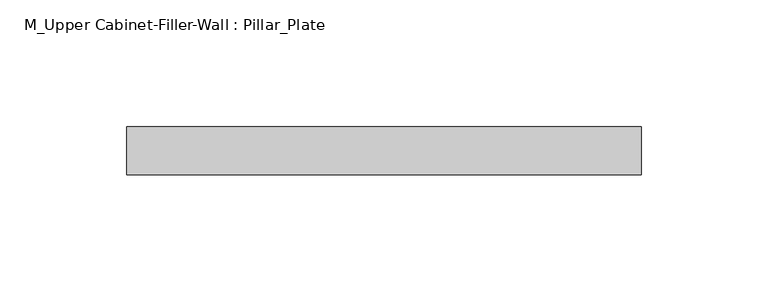
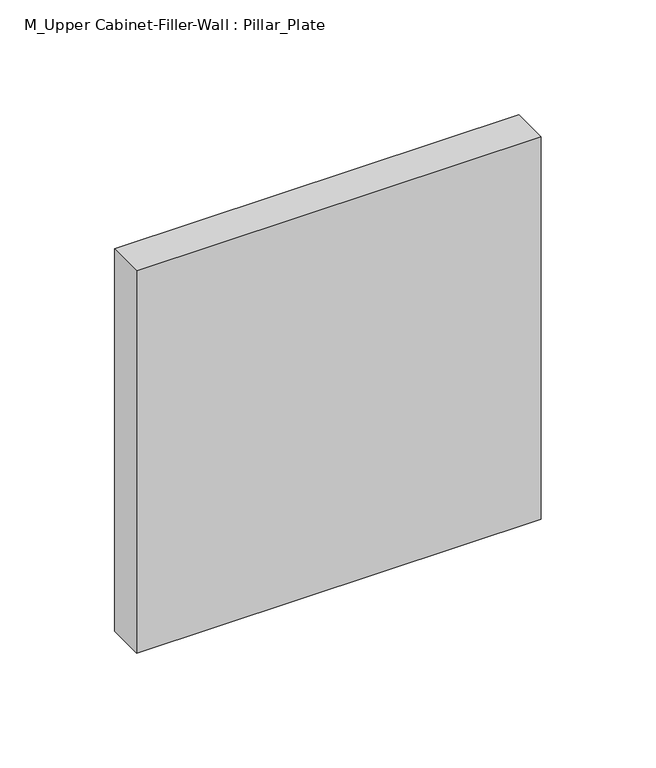
"""IFC4 building model written with IfcOpenShell, lengths in millimetres: furniture geometry, M_Upper Cabinet-Filler-Wall : Pillar_Plate."""

from ifc_helpers import new_model, si_unit, frame, origin, place, context, project, spatial, polyline, outline, extrude, source, transform, mapped, element, save


def m_upper_cabinet_filler_wall_pillar_plate_184ded32(model_context):
    return source(origin(), model_context, "Body", "SweptSolid", [
        extrude(outline(polyline([(-71.8288372, 38.1), (-71.8288372, 57.15), (131.3711628, 57.15), (131.3711628, 38.1), (-71.8288372, 38.1)])), frame((0.0, 0.0, 1796.8), z_axis=(0.0, 0.0, 1.0), x_axis=(1.0, 0.0, 0.0)), (0.0, 0.0, 1.0), 203.2),
    ])


if __name__ == "__main__":
    model = new_model("IFC4")
    model_context = context("Model", 3, world=origin())
    ifc_project = project(units=[si_unit("LENGTHUNIT", "METRE", prefix="MILLI")], contexts=[model_context])
    site = spatial("IfcSite", under=ifc_project)
    building = spatial("IfcBuilding", under=site)
    placement = place(None, origin())
    m_upper_cabinet_filler_wall_pillar_plate_shape = m_upper_cabinet_filler_wall_pillar_plate_184ded32(model_context)
    element("IfcFurniture", 1, ObjectType="M_Upper Cabinet-Filler-Wall : Pillar_Plate", at=placement, inside=building, context=model_context, shape_type="MappedRepresentation", body=[
        mapped(m_upper_cabinet_filler_wall_pillar_plate_shape, transform((0.0, 0.0, 0.0), x_axis=(1.0, 0.0, 0.0), y_axis=(0.0, 1.0, 0.0), z_axis=(0.0, 0.0, 1.0))),
    ])
    save(model, "model.ifc")

# Revit data of these elements
# Type "M_Upper Cabinet-Filler-Wall : Pillar_Plate"
#   Depth = 0' - 1"
#   Height = 0' - 8"
#   Top Of Cabinet = 6' - 6.74016"
#   Width = 0' - 8"
#   Cabinet Material = none
#   Default Elevation = 0
# Element 1 (IfcFurniture, "M_Upper Cabinet-Filler-Wall : Pillar_Plate")
#   Materials on its faces: "Cabinets"
# Materials
#   "Cabinets": class "Miscellaneous", colour RGB 249 249 249, transparency 0
